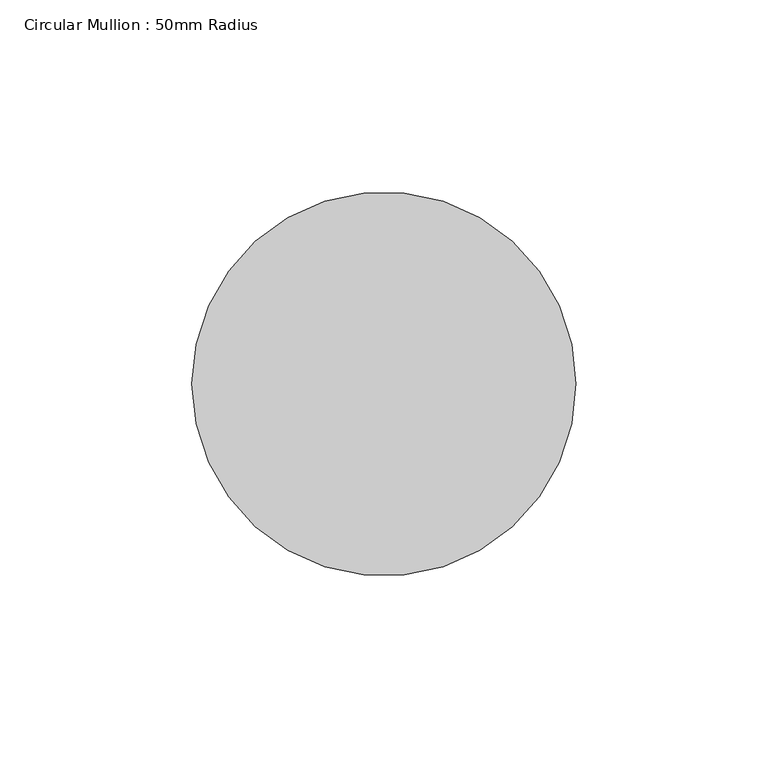
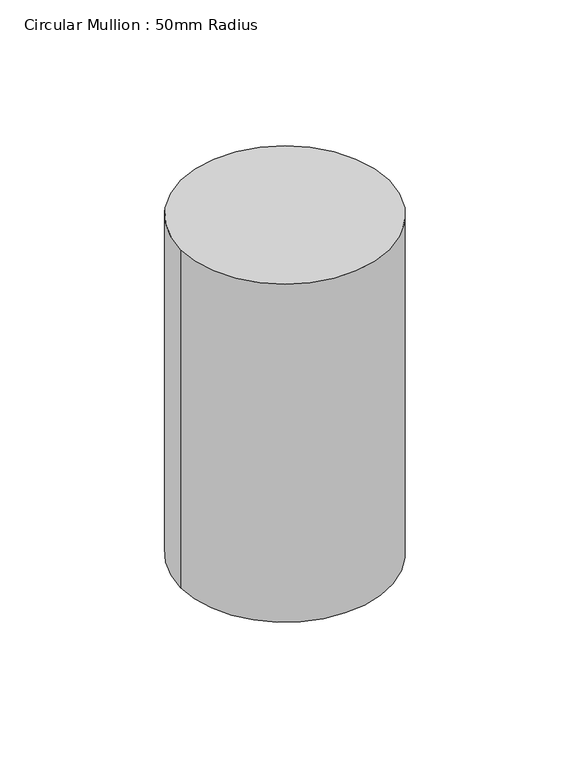
"""IFC4 building model written with IfcOpenShell, lengths in millimetres: member geometry, Circular Mullion : 50mm Radius."""

from ifc_helpers import new_model, si_unit, point, frame, origin, origin_2d, place, context, project, spatial, circle_curve, trimmed, segment, composite_curve, outline, extrude, source, transform, mapped, element, save


def circular_mullion_50mm_radius_fa87843c(model_context):
    return source(origin(), model_context, "Body", "SweptSolid", [
        extrude(outline(composite_curve([segment(trimmed(circle_curve(origin_2d(), 50.0), [point((50.0, 0.0))], [point((-50.0, 0.0))], False, "CARTESIAN"), True, "CONTINUOUS"), segment(trimmed(circle_curve(origin_2d(), 50.0), [point((-50.0, 0.0))], [point((50.0, 0.0))], False, "CARTESIAN"), True, "CONTINUOUS")], self_intersect=False)), frame((0.0, 0.0, -171.2308041), z_axis=(0.0, 0.0, 1.0), x_axis=(1.0, 0.0, 0.0)), (0.0, 0.0, 1.0), 171.2308041),
    ])


if __name__ == "__main__":
    model = new_model("IFC4")
    model_context = context("Model", 3, world=origin())
    ifc_project = project(units=[si_unit("LENGTHUNIT", "METRE", prefix="MILLI")], contexts=[model_context])
    site = spatial("IfcSite", under=ifc_project)
    building = spatial("IfcBuilding", under=site)
    placement = place(None, origin())
    circular_mullion_50mm_radius_shape = circular_mullion_50mm_radius_fa87843c(model_context)
    element("IfcMember", 1, ObjectType="Circular Mullion : 50mm Radius", at=placement, inside=building, context=model_context, shape_type="MappedRepresentation", body=[
        mapped(circular_mullion_50mm_radius_shape, transform((0.0, 0.0, 0.0), x_axis=(1.0, 0.0, 0.0), y_axis=(0.0, 1.0, 0.0), z_axis=(0.0, 0.0, 1.0))),
    ])
    save(model, "model.ifc")

# Revit data of these elements
# Type "Circular Mullion : 50mm Radius"
#   built-in parameter 1007350 = 0.164042 (stored number, unit not read)
# Element 1 (IfcMember, "Circular Mullion : 50mm Radius")
#   Materials on its faces: "Aluminium"
# Materials
#   "Aluminium": class "Metal", colour RGB 247 247 247, transparency 0, Description = "Aluminium 6061", Cost = 0
